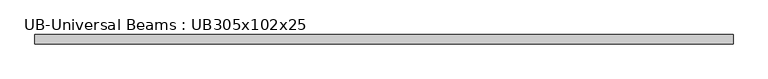
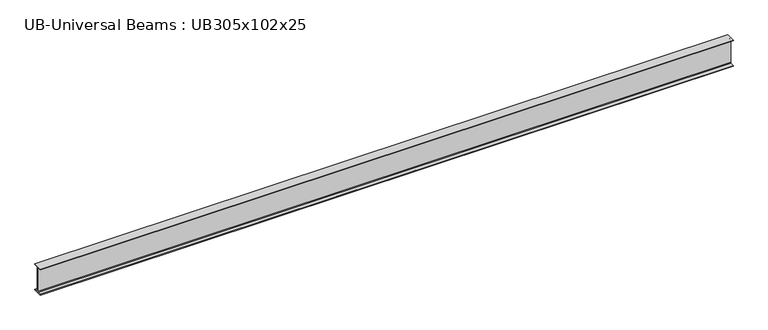
"""IFC4 building model written with IfcOpenShell, lengths in millimetres: beam geometry, UB-Universal Beams : UB305x102x25."""

from ifc_helpers import new_model, si_unit, point, frame, frame_2d, origin, place, context, project, spatial, polyline, circle_curve, trimmed, segment, composite_curve, outline, extrude, source, transform, mapped, element, save


def ub_universal_beams_ub305x102x25_ce7b4b23(model_context):
    return source(origin(), model_context, "Body", "SweptSolid", [
        extrude(outline(composite_curve([segment(polyline([(50.8, -145.55), (50.8, -152.55), (-50.8, -152.55), (-50.8, -145.55), (-10.5, -145.55)]), True, "CONTINUOUS"), segment(trimmed(circle_curve(frame_2d((-10.5, -137.95)), 7.6), [point((-10.5, -145.55))], [point((-2.9, -137.95))], True, "CARTESIAN"), True, "CONTINUOUS"), segment(polyline([(-2.9, -137.95), (-2.9, 137.95)]), True, "CONTINUOUS"), segment(trimmed(circle_curve(frame_2d((-10.5, 137.95)), 7.6), [point((-2.9, 137.95))], [point((-10.5, 145.55))], True, "CARTESIAN"), True, "CONTINUOUS"), segment(polyline([(-10.5, 145.55), (-50.8, 145.55), (-50.8, 152.55), (50.8, 152.55), (50.8, 145.55), (10.5, 145.55)]), True, "CONTINUOUS"), segment(trimmed(circle_curve(frame_2d((10.5, 137.95)), 7.6), [point((10.5, 145.55))], [point((2.9, 137.95))], True, "CARTESIAN"), True, "CONTINUOUS"), segment(polyline([(2.9, 137.95), (2.9, -137.95)]), True, "CONTINUOUS"), segment(trimmed(circle_curve(frame_2d((10.5, -137.95)), 7.6), [point((2.9, -137.95))], [point((10.5, -145.55))], True, "CARTESIAN"), True, "CONTINUOUS"), segment(polyline([(10.5, -145.55), (50.8, -145.55)]), True, "CONTINUOUS")], self_intersect=False)), frame((-3850.0, 0.0, 0.0), z_axis=(1.0, 0.0, 0.0), x_axis=(0.0, 1.0, 0.0)), (0.0, 0.0, 1.0), 7700.0),
    ])


if __name__ == "__main__":
    model = new_model("IFC4")
    model_context = context("Model", 3, world=origin())
    ifc_project = project(units=[si_unit("LENGTHUNIT", "METRE", prefix="MILLI")], contexts=[model_context])
    site = spatial("IfcSite", under=ifc_project)
    building = spatial("IfcBuilding", under=site)
    placement = place(None, origin())
    ub_universal_beams_ub305x102x25_shape = ub_universal_beams_ub305x102x25_ce7b4b23(model_context)
    element("IfcBeam", 1, ObjectType="UB-Universal Beams : UB305x102x25", at=placement, inside=building, context=model_context, shape_type="MappedRepresentation", body=[
        mapped(ub_universal_beams_ub305x102x25_shape, transform((0.0, 0.0, 0.0), x_axis=(1.0, 0.0, 0.0), y_axis=(0.0, 1.0, 0.0), z_axis=(0.0, 0.0, 1.0))),
    ])
    save(model, "model.ifc")

# Revit data of these elements
# Type "UB-Universal Beams : UB305x102x25"
#   Section Name Key = "UB305X102X25"
#   Width = 10.16 cm
#   Web Thickness = 0.58 cm
#   Web Fillet = 0.76 cm
#   Warping Constant = 27300.0 cm⁶
#   Torsional Moment of Inertia = 4.77 cm⁴
#   Section Area = 31.6 cm²
#   Plastic Modulus weak axis = 39.0 cm³
#   Plastic Modulus strong axis = 342.0 cm³
#   Nominal Weight = 24.7999 kgf/m
#   Moment of Inertia weak axis = 123.00 cm⁴
#   Moment of Inertia strong axis = 4455.00 cm⁴
#   Height = 30.51 cm
#   Flange Thickness = 0.7 cm
#   Elastic Modulus weak axis = 24.2 cm³
#   Elastic Modulus strong axis = 292.0 cm³
#   Centroid Vertical = 15.255 cm
#   Centroid Horizontal = 5.08 cm
#   Bolt Spacing = 5.4 cm
#   Length [instance default] = 1500 mm
#   Structural Material [instance default] = Metal - Steel 43-275
#   Type Comments = ""
#   Assembly Code = ""
# Element 1 (IfcBeam, "UB-Universal Beams : UB305x102x25")
#   Materials on its faces: "Metal - Steel 43-275"
# Materials
#   "Metal - Steel 43-275": class "Metal", colour RGB 247 247 247, transparency 0, Cost = 0
